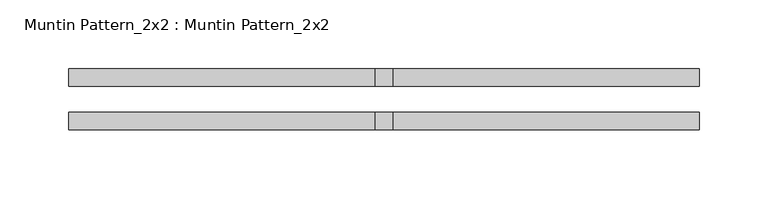
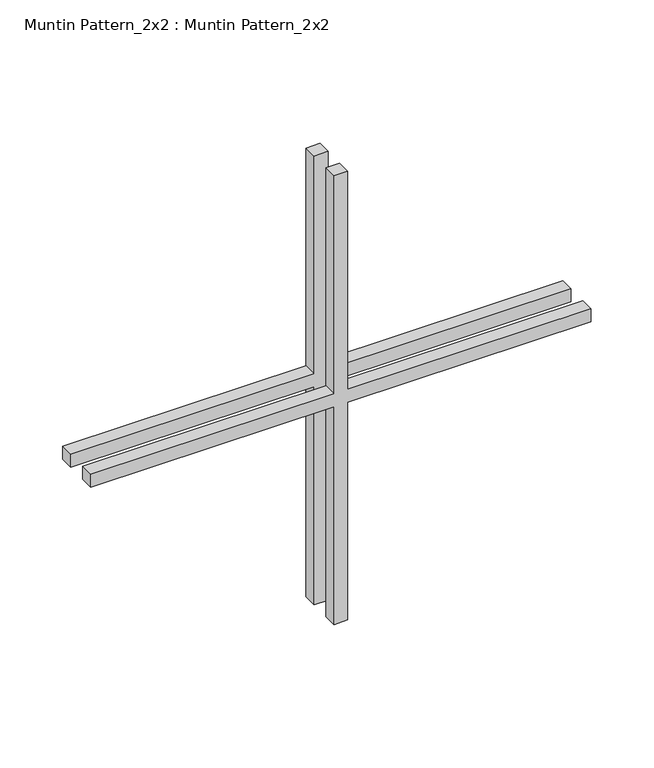
"""IFC4 building model written with IfcOpenShell, lengths in millimetres: proxy geometry, Muntin Pattern_2x2 : Muntin Pattern_2x2."""

from ifc_helpers import new_model, si_unit, frame, origin, place, context, project, spatial, polyline, outline, extrude, source, transform, mapped, element, save


def muntin_pattern_2x2_muntin_pattern_2x2_c59e45a7(model_context):
    return source(origin(), model_context, "Body", "SweptSolid", [
        extrude(outline(polyline([(223.8375, -6.35), (223.8375, -229.39375), (211.1375, -229.39375), (211.1375, -6.35), (0.0, -6.35), (0.0, 6.35), (211.1375, 6.35), (211.1375, 229.39375), (223.8375, 229.39375), (223.8375, 6.35), (434.975, 6.35), (434.975, -6.35), (223.8375, -6.35)])), frame((0.0, 9.525, 0.0), z_axis=(0.0, 1.0, 0.0), x_axis=(0.0, 0.0, 1.0)), (0.0, 0.0, 1.0), 12.7),
        extrude(outline(polyline([(223.8375, -6.35), (223.8375, -229.39375), (211.1375, -229.39375), (211.1375, -6.35), (0.0, -6.35), (0.0, 6.35), (211.1375, 6.35), (211.1375, 229.39375), (223.8375, 229.39375), (223.8375, 6.35), (434.975, 6.35), (434.975, -6.35), (223.8375, -6.35)])), frame((0.0, -22.225, 0.0), z_axis=(0.0, 1.0, 0.0), x_axis=(0.0, 0.0, 1.0)), (0.0, 0.0, 1.0), 12.7),
    ])


if __name__ == "__main__":
    model = new_model("IFC4")
    model_context = context("Model", 3, world=origin())
    ifc_project = project(units=[si_unit("LENGTHUNIT", "METRE", prefix="MILLI")], contexts=[model_context])
    site = spatial("IfcSite", under=ifc_project)
    building = spatial("IfcBuilding", under=site)
    placement = place(None, origin())
    muntin_pattern_2x2_muntin_pattern_2x2_shape = muntin_pattern_2x2_muntin_pattern_2x2_c59e45a7(model_context)
    element("IfcBuildingElementProxy", 1, Name="Muntin Pattern_2x2 : Muntin Pattern_2x2", ObjectType="Muntin Pattern_2x2 : Muntin Pattern_2x2", at=placement, inside=building, context=model_context, shape_type="MappedRepresentation", body=[
        mapped(muntin_pattern_2x2_muntin_pattern_2x2_shape, transform((0.0, 0.0, 0.0), x_axis=(1.0, 0.0, 0.0), y_axis=(0.0, 1.0, 0.0), z_axis=(0.0, 0.0, 1.0))),
    ])
    save(model, "model.ifc")

# Revit data of these elements
# Type "Muntin Pattern_2x2 : Muntin Pattern_2x2"
#   Width [instance default] = 121.92 cm
#   Thickness = 1.27 cm
#   Height [instance default] = 121.92 cm
#   Distance = 1.905 cm
#   Interior Material [instance default] = none
#   Exterior Material [instance default] = none
# Element 1 (IfcBuildingElementProxy, "Muntin Pattern_2x2 : Muntin Pattern_2x2")
#   Width = 45.8787 cm
#   Height = 43.4975 cm
#   Interior Material = Wood - Stained
#   Exterior Material = Clad - White
#   Materials on its faces: "Clad - White", "Wood - Stained"
# Materials
#   "Clad - White": class "Wood", colour RGB 242 242 238, transparency 0, Cost = 0
#   "Wood - Stained": class "Wood", colour RGB 224 178 126, transparency 0, Cost = 0
